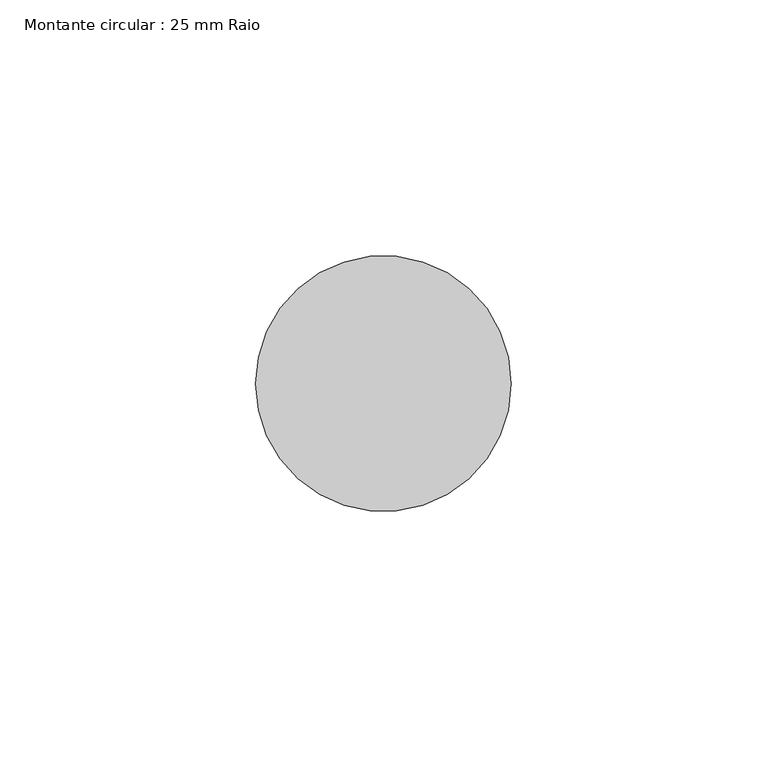
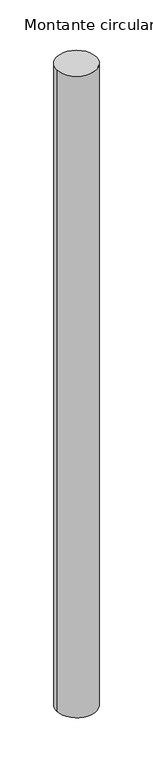
"""IFC4 building model written with IfcOpenShell, lengths in millimetres: member geometry, Montante circular : 25 mm Raio."""

import ifcopenshell
import ifcopenshell.guid

model = None  # the IFC model being written
_history = None  # IfcOwnerHistory: only IFC2X3 demands one
_inside = {}  # id of a spatial element -> (the spatial element, [elements in it])
_under = {}  # id of a project, library or spatial element -> (it, [spatial elements below it])
_declared = {}  # id of a project -> (the project, [libraries it declares])
_typed = {}  # id of a type object -> (the type object, [elements of that type])
_made_of = {}  # id of a material, layer set ... -> (it, [elements and type objects made of it])


def new_model(schema):
    """Start an empty IFC model of exactly this schema.

    Asked for "IFC4X3", IfcOpenShell would pick the latest addendum, in which some entities
    have other attributes; the version numbers below select the first issue.
    IFC2X3 requires an IfcOwnerHistory on every rooted entity: one is made here for all.
    """
    global model, _history
    if schema == "IFC4X3":
        model = ifcopenshell.file(schema_version=(4, 3, 0, 0))
    else:
        model = ifcopenshell.file(schema=schema)
    _inside.clear()
    _under.clear()
    _declared.clear()
    _typed.clear()
    _made_of.clear()
    _history = None
    if model.schema == "IFC2X3":
        org = make("IfcOrganization", Name="unknown")
        user = make(
            "IfcPersonAndOrganization",
            ThePerson=make("IfcPerson", FamilyName="unknown"),
            TheOrganization=org,
        )
        app = make(
            "IfcApplication",
            ApplicationDeveloper=org,
            Version="unknown",
            ApplicationFullName="unknown",
            ApplicationIdentifier="unknown",
        )
        _history = make(
            "IfcOwnerHistory",
            OwningUser=user,
            OwningApplication=app,
            ChangeAction="ADDED",
            CreationDate=0,
        )
    return model


def make(cls, **values):
    """One entity of the class cls with the attributes given. An attribute that is None is left unset."""
    return model.create_entity(
        cls, **{name: value for name, value in values.items() if value is not None}
    )


def rooted(cls, **values):
    """An entity with a GlobalId (a new one), such as an element, a storey or a relation."""
    return make(cls, GlobalId=ifcopenshell.guid.new(), OwnerHistory=_history, **values)


def si_unit(unit_type, name, prefix=None):
    """IfcSIUnit, for example si_unit("LENGTHUNIT", "METRE", prefix="MILLI")."""
    return make("IfcSIUnit", UnitType=unit_type, Prefix=prefix, Name=name)


def assignment(units):
    """IfcUnitAssignment: the units of a project."""
    return None if units is None else make("IfcUnitAssignment", Units=units)


def point(xyz):
    """IfcCartesianPoint."""
    return None if xyz is None else make("IfcCartesianPoint", Coordinates=xyz)


def direction(xyz):
    """IfcDirection."""
    return None if xyz is None else make("IfcDirection", DirectionRatios=xyz)


def frame(location, z_axis=None, x_axis=None):
    """IfcAxis2Placement3D, a coordinate frame: its origin and axes. An axis left out is left unset."""
    return make(
        "IfcAxis2Placement3D",
        Location=point(location),
        Axis=direction(z_axis),
        RefDirection=direction(x_axis),
    )


def frame_2d(location, x_axis=None):
    """IfcAxis2Placement2D, a coordinate frame in the plane: its origin and x axis."""
    return make(
        "IfcAxis2Placement2D", Location=point(location), RefDirection=direction(x_axis)
    )


def origin():
    """The frame at (0, 0, 0) with its axes left unset."""
    return frame((0.0, 0.0, 0.0))


def origin_2d():
    """The frame at (0, 0) in the plane with its x axis left unset."""
    return frame_2d((0.0, 0.0))


def place(relative_to, where):
    """IfcLocalPlacement: puts the frame where relative to a parent placement (None: the world)."""
    return make(
        "IfcLocalPlacement", PlacementRelTo=relative_to, RelativePlacement=where
    )


def context(
    kind, dimensions, precision=None, world=None, true_north=None, identifier=None
):
    """IfcGeometricRepresentationContext, for example the 3D "Model" context."""
    return make(
        "IfcGeometricRepresentationContext",
        ContextIdentifier=identifier,
        ContextType=kind,
        CoordinateSpaceDimension=dimensions,
        Precision=precision,
        WorldCoordinateSystem=world,
        TrueNorth=true_north,
    )


def project(units=None, contexts=None):
    """IfcProject with its units and contexts."""
    return rooted(
        "IfcProject",
        Name="project",
        RepresentationContexts=contexts,
        UnitsInContext=assignment(units),
    )


def spatial(cls, under=None, at=None, **own):
    """A site, building, storey or space (cls), placed at a placement, below another one or the project."""
    s = rooted(cls, ObjectPlacement=at, **own)
    if under is not None:
        _under.setdefault(under.id(), (under, []))[1].append(s)
    return s


def circle_curve(where, radius):
    """IfcCircle in the frame where."""
    return make("IfcCircle", Position=where, Radius=radius)


def trimmed(basis, trim1, trim2, sense, master):
    """IfcTrimmedCurve: the piece of a basis curve between two trims."""
    return make(
        "IfcTrimmedCurve",
        BasisCurve=basis,
        Trim1=trim1,
        Trim2=trim2,
        SenseAgreement=sense,
        MasterRepresentation=master,
    )


def segment(curve, same_sense, transition):
    """IfcCompositeCurveSegment."""
    return make(
        "IfcCompositeCurveSegment",
        Transition=transition,
        SameSense=same_sense,
        ParentCurve=curve,
    )


def composite_curve(segments, self_intersect=None):
    """IfcCompositeCurve: segments joined end to end."""
    return make("IfcCompositeCurve", Segments=segments, SelfIntersect=self_intersect)


def outline(outer, holes=None, kind="AREA"):
    """IfcArbitraryClosedProfileDef: a profile drawn as a closed curve; with holes, ...WithVoids."""
    if holes is None:
        return make("IfcArbitraryClosedProfileDef", ProfileType=kind, OuterCurve=outer)
    return make(
        "IfcArbitraryProfileDefWithVoids",
        ProfileType=kind,
        OuterCurve=outer,
        InnerCurves=holes,
    )


def extrude(swept, where, along, depth):
    """IfcExtrudedAreaSolid: the profile swept, set in the frame where, extruded along a direction by depth."""
    return make(
        "IfcExtrudedAreaSolid",
        SweptArea=swept,
        Position=where,
        ExtrudedDirection=direction(along),
        Depth=depth,
    )


def shape(context_of_items, identifier, shape_type, items):
    """IfcShapeRepresentation: the items that make up one representation, for example the "Body"."""
    return make(
        "IfcShapeRepresentation",
        ContextOfItems=context_of_items,
        RepresentationIdentifier=identifier,
        RepresentationType=shape_type,
        Items=items,
    )


def source(mapping_origin, context_of_items, identifier, shape_type, items):
    """IfcRepresentationMap: a shape defined once, which mapped items show again and again."""
    return make(
        "IfcRepresentationMap",
        MappingOrigin=mapping_origin,
        MappedRepresentation=shape(context_of_items, identifier, shape_type, items),
    )


def transform(
    local_origin,
    x_axis=None,
    y_axis=None,
    z_axis=None,
    scale=None,
    scale2=None,
    scale3=None,
    uniform=True,
):
    """IfcCartesianTransformationOperator3D, or its non-uniform kind. x_axis, y_axis, z_axis: its Axis1, 2, 3."""
    if uniform:
        return make(
            "IfcCartesianTransformationOperator3D",
            Axis1=direction(x_axis),
            Axis2=direction(y_axis),
            LocalOrigin=point(local_origin),
            Scale=scale,
            Axis3=direction(z_axis),
        )
    return make(
        "IfcCartesianTransformationOperator3DnonUniform",
        Axis1=direction(x_axis),
        Axis2=direction(y_axis),
        LocalOrigin=point(local_origin),
        Scale=scale,
        Axis3=direction(z_axis),
        Scale2=scale2,
        Scale3=scale3,
    )


def mapped(mapping_source, mapping_target):
    """IfcMappedItem: shows the shape of a source again, moved by a transform."""
    return make(
        "IfcMappedItem", MappingSource=mapping_source, MappingTarget=mapping_target
    )


def made_of(thing, what):
    """Note that an element or type object is made of a material, layer set ...; save() writes the relation."""
    if what is not None:
        _made_of.setdefault(what.id(), (what, []))[1].append(thing)
    return thing


def element(
    cls,
    number,
    at=None,
    inside=None,
    cuts=None,
    type_object=None,
    material=None,
    context=None,
    identifier="Body",
    shape_type=None,
    held_by="IfcProductDefinitionShape",
    body=None,
    shapes=None,
    **own,
):
    """One element of the class cls, such as IfcWall. Its Tag is "e" and its number.

    at: its placement. inside: the storey or other place that contains it. cuts: it is an
    opening in that element (IfcRelVoidsElement). A single representation is given by context,
    identifier, shape_type and body (its items); several are given by shapes. held_by: the class
    of the entity that holds the representations. save() writes the other relations.
    """
    e = rooted(cls, Tag="e%d" % number, ObjectPlacement=at, **own)
    if body is not None:
        shapes = [shape(context, identifier, shape_type, body)]
    if shapes is not None:
        e.Representation = make(held_by, Representations=shapes)
    if inside is not None:
        _inside.setdefault(inside.id(), (inside, []))[1].append(e)
    if cuts is not None:
        rooted(
            "IfcRelVoidsElement", RelatingBuildingElement=cuts, RelatedOpeningElement=e
        )
    if type_object is not None:
        _typed.setdefault(type_object.id(), (type_object, []))[1].append(e)
    return made_of(e, material)


def aggregate(whole, parts):
    """IfcRelAggregates: a whole, such as a stair, and the parts it consists of."""
    return rooted("IfcRelAggregates", RelatingObject=whole, RelatedObjects=parts)


def save(model, path):
    """Write the relations noted so far, then the file.

    IfcRelAggregates (storeys below a building ...), IfcRelContainedInSpatialStructure (elements
    in a storey), IfcRelDefinesByType, IfcRelAssociatesMaterial and IfcRelDeclares: one each for
    every whole, place, type object, material and project.
    """
    for whole, parts in _under.values():
        aggregate(whole, parts)
    for where, things in _inside.values():
        rooted(
            "IfcRelContainedInSpatialStructure",
            RelatedElements=things,
            RelatingStructure=where,
        )
    for kind, things in _typed.values():
        rooted("IfcRelDefinesByType", RelatedObjects=things, RelatingType=kind)
    for what, things in _made_of.values():
        rooted("IfcRelAssociatesMaterial", RelatedObjects=things, RelatingMaterial=what)
    for by, libraries in _declared.values():
        rooted("IfcRelDeclares", RelatingContext=by, RelatedDefinitions=libraries)
    model.write(path)


def montante_circular_25_mm_raio_855f7cf8(model_context):
    return source(origin(), model_context, "Body", "SweptSolid", [
        extrude(outline(composite_curve([segment(trimmed(circle_curve(origin_2d(), 25.0), [point((25.0, 0.0))], [point((-25.0, 0.0))], False, "CARTESIAN"), True, "CONTINUOUS"), segment(trimmed(circle_curve(origin_2d(), 25.0), [point((-25.0, 0.0))], [point((25.0, 0.0))], False, "CARTESIAN"), True, "CONTINUOUS")], self_intersect=False)), frame((0.0, 0.0, -861.4383425), z_axis=(0.0, 0.0, 1.0), x_axis=(1.0, 0.0, 0.0)), (0.0, 0.0, 1.0), 861.4383425),
    ])


if __name__ == "__main__":
    model = new_model("IFC4")
    model_context = context("Model", 3, world=origin())
    ifc_project = project(units=[si_unit("LENGTHUNIT", "METRE", prefix="MILLI")], contexts=[model_context])
    site = spatial("IfcSite", under=ifc_project)
    building = spatial("IfcBuilding", under=site)
    placement = place(None, origin())
    montante_circular_25_mm_raio_shape = montante_circular_25_mm_raio_855f7cf8(model_context)
    element("IfcMember", 1, ObjectType="Montante circular : 25 mm Raio", at=placement, inside=building, context=model_context, shape_type="MappedRepresentation", body=[
        mapped(montante_circular_25_mm_raio_shape, transform((0.0, 0.0, 0.0), x_axis=(1.0, 0.0, 0.0), y_axis=(0.0, 1.0, 0.0), z_axis=(0.0, 0.0, 1.0))),
    ])
    save(model, "model.ifc")

# Revit data of these elements
# Type "Montante circular : 25 mm Raio"
#   built-in parameter 1007350 = 0.082021 (stored number, unit not read)
# Element 1 (IfcMember, "Montante circular : 25 mm Raio")
#   Materials on its faces: "Alumín."
# Materials
#   "Alumín.": class "Metal", colour RGB 247 247 247, transparency 0, Description = "Alumín. 6061", Cost = 0
